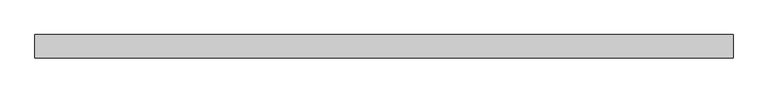
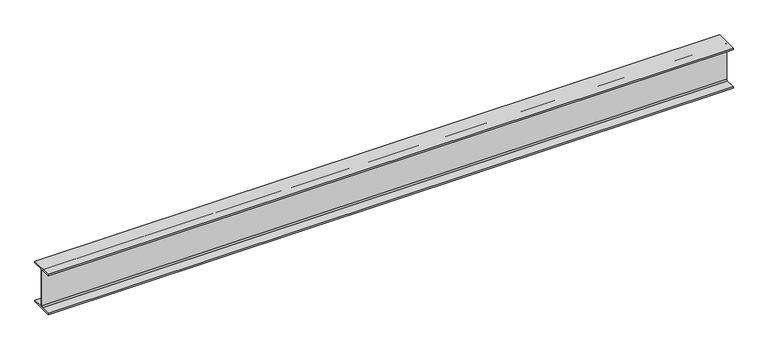
"""IFC4 building model written with IfcOpenShell, lengths in millimetres: beam geometry, Old_Steel Beam_H-KSD3502 : H_SB_ASB_H-300×300x10x15."""

from ifc_helpers import new_model, si_unit, point, frame, frame_2d, origin, place, context, project, spatial, polyline, circle_curve, trimmed, segment, composite_curve, outline, extrude, source, transform, mapped, element, save


def beam_952dd806(model_context):
    return source(origin(), model_context, "Body", "SweptSolid", [
        extrude(outline(composite_curve([segment(polyline([(-82.5, -141.5), (-11.9, -141.5)]), True, "CONTINUOUS"), segment(trimmed(circle_curve(frame_2d((-11.9, -132.6)), 8.9), [point((-11.9, -141.5))], [point((-3.0, -132.6))], True, "CARTESIAN"), True, "CONTINUOUS"), segment(polyline([(-3.0, -132.6), (-3.0, 132.6)]), True, "CONTINUOUS"), segment(trimmed(circle_curve(frame_2d((-11.9, 132.6)), 8.9), [point((-3.0, 132.6))], [point((-11.9, 141.5))], True, "CARTESIAN"), True, "CONTINUOUS"), segment(polyline([(-11.9, 141.5), (-82.5, 141.5), (-82.5, 151.7), (82.5, 151.7), (82.5, 141.5), (11.9, 141.5)]), True, "CONTINUOUS"), segment(trimmed(circle_curve(frame_2d((11.9, 132.6)), 8.9), [point((11.9, 141.5))], [point((3.0, 132.6))], True, "CARTESIAN"), True, "CONTINUOUS"), segment(polyline([(3.0, 132.6), (3.0, -132.6)]), True, "CONTINUOUS"), segment(trimmed(circle_curve(frame_2d((11.9, -132.6)), 8.9), [point((3.0, -132.6))], [point((11.9, -141.5))], True, "CARTESIAN"), True, "CONTINUOUS"), segment(polyline([(11.9, -141.5), (82.5, -141.5), (82.5, -151.7), (-82.5, -151.7), (-82.5, -141.5)]), True, "CONTINUOUS")], self_intersect=False)), frame((-2479.7628546, 0.0, 0.0), z_axis=(1.0, 0.0, 0.0), x_axis=(0.0, 1.0, 0.0)), (0.0, 0.0, 1.0), 4891.0868037),
    ])


if __name__ == "__main__":
    model = new_model("IFC4")
    model_context = context("Model", 3, world=origin())
    ifc_project = project(units=[si_unit("LENGTHUNIT", "METRE", prefix="MILLI")], contexts=[model_context])
    site = spatial("IfcSite", under=ifc_project)
    building = spatial("IfcBuilding", under=site)
    placement = place(None, origin())
    beam_shape = beam_952dd806(model_context)
    element("IfcBeam", 1, ObjectType="Old_Steel Beam_H-KSD3502 : H_SB_ASB_H-300×300x10x15", at=placement, inside=building, context=model_context, shape_type="MappedRepresentation", body=[
        mapped(beam_shape, transform((0.0, 0.0, 0.0), x_axis=(1.0, 0.0, 0.0), y_axis=(0.0, 1.0, 0.0), z_axis=(0.0, 0.0, 1.0))),
    ])
    save(model, "model.ifc")

# Revit data of these elements
# Type "Old_Steel Beam_H-KSD3502 : H_SB_ASB_H-300×300x10x15"
#   Width = 30.0 cm
#   Web Thickness = 1.0 cm
#   Web Fillet = 1.8 cm
#   Warping Constant = 1370670.0 cm⁶
#   Torsional Moment of Inertia = 77.00 cm⁴
#   Torsional Modulus = 1.0 cm³
#   Section Area = 119.8 cm²
#   Plastic Modulus weak axis = 684.0 cm³
#   Plastic Modulus strong axis = 1500.0 cm³
#   Perimeter = 1.75 m²/m
#   Nominal Weight = 94.00 kgf/m
#   Moment of Inertia weak axis = 6750.00 cm⁴
#   Moment of Inertia strong axis = 20400.00 cm⁴
#   Height = 30.0 cm
#   Flange Thickness = 1.5 cm
#   Elastic Modulus weak axis = 450.0 cm³
#   Elastic Modulus strong axis = 1360.0 cm³
#   Centroid Vertical = 15.0 cm
#   Centroid Horizontal = 15.0 cm
#   Length [instance default] = 1.5240 m
#   Structural Material [instance default] = Steel, 45-345
#   Assembly Code = ""
# Element 1 (IfcBeam, "Old_Steel Beam_H-KSD3502 : H_SB_ASB_H-300×300x10x15")
#   Structural Material = none
# Materials
#   "Steel, 45-345": class "Metal", colour RGB 189 187 185, transparency 0, Description = "Steel 345 MPa", Cost = 0
